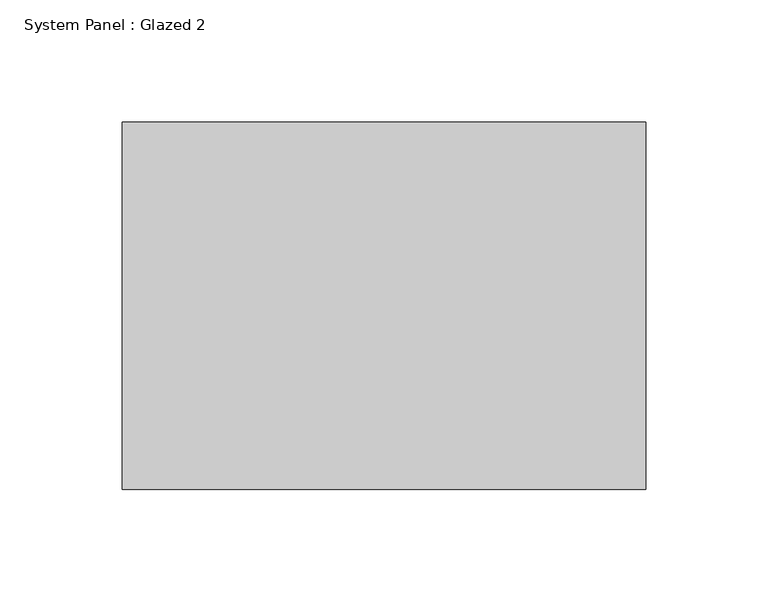
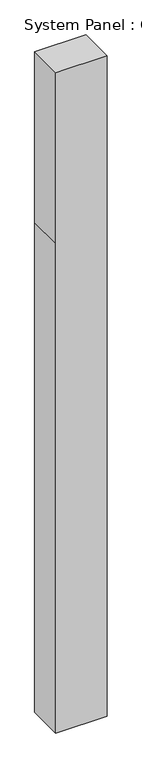
"""IFC4 building model written with IfcOpenShell, lengths in millimetres: plate geometry, System Panel : Glazed 2."""

import ifcopenshell
import ifcopenshell.guid

model = None  # the IFC model being written
_history = None  # IfcOwnerHistory: only IFC2X3 demands one
_inside = {}  # id of a spatial element -> (the spatial element, [elements in it])
_under = {}  # id of a project, library or spatial element -> (it, [spatial elements below it])
_declared = {}  # id of a project -> (the project, [libraries it declares])
_typed = {}  # id of a type object -> (the type object, [elements of that type])
_made_of = {}  # id of a material, layer set ... -> (it, [elements and type objects made of it])


def new_model(schema):
    """Start an empty IFC model of exactly this schema.

    Asked for "IFC4X3", IfcOpenShell would pick the latest addendum, in which some entities
    have other attributes; the version numbers below select the first issue.
    IFC2X3 requires an IfcOwnerHistory on every rooted entity: one is made here for all.
    """
    global model, _history
    if schema == "IFC4X3":
        model = ifcopenshell.file(schema_version=(4, 3, 0, 0))
    else:
        model = ifcopenshell.file(schema=schema)
    _inside.clear()
    _under.clear()
    _declared.clear()
    _typed.clear()
    _made_of.clear()
    _history = None
    if model.schema == "IFC2X3":
        org = make("IfcOrganization", Name="unknown")
        user = make(
            "IfcPersonAndOrganization",
            ThePerson=make("IfcPerson", FamilyName="unknown"),
            TheOrganization=org,
        )
        app = make(
            "IfcApplication",
            ApplicationDeveloper=org,
            Version="unknown",
            ApplicationFullName="unknown",
            ApplicationIdentifier="unknown",
        )
        _history = make(
            "IfcOwnerHistory",
            OwningUser=user,
            OwningApplication=app,
            ChangeAction="ADDED",
            CreationDate=0,
        )
    return model


def make(cls, **values):
    """One entity of the class cls with the attributes given. An attribute that is None is left unset."""
    return model.create_entity(
        cls, **{name: value for name, value in values.items() if value is not None}
    )


def rooted(cls, **values):
    """An entity with a GlobalId (a new one), such as an element, a storey or a relation."""
    return make(cls, GlobalId=ifcopenshell.guid.new(), OwnerHistory=_history, **values)


def si_unit(unit_type, name, prefix=None):
    """IfcSIUnit, for example si_unit("LENGTHUNIT", "METRE", prefix="MILLI")."""
    return make("IfcSIUnit", UnitType=unit_type, Prefix=prefix, Name=name)


def assignment(units):
    """IfcUnitAssignment: the units of a project."""
    return None if units is None else make("IfcUnitAssignment", Units=units)


def point(xyz):
    """IfcCartesianPoint."""
    return None if xyz is None else make("IfcCartesianPoint", Coordinates=xyz)


def direction(xyz):
    """IfcDirection."""
    return None if xyz is None else make("IfcDirection", DirectionRatios=xyz)


def frame(location, z_axis=None, x_axis=None):
    """IfcAxis2Placement3D, a coordinate frame: its origin and axes. An axis left out is left unset."""
    return make(
        "IfcAxis2Placement3D",
        Location=point(location),
        Axis=direction(z_axis),
        RefDirection=direction(x_axis),
    )


def origin():
    """The frame at (0, 0, 0) with its axes left unset."""
    return frame((0.0, 0.0, 0.0))


def place(relative_to, where):
    """IfcLocalPlacement: puts the frame where relative to a parent placement (None: the world)."""
    return make(
        "IfcLocalPlacement", PlacementRelTo=relative_to, RelativePlacement=where
    )


def context(
    kind, dimensions, precision=None, world=None, true_north=None, identifier=None
):
    """IfcGeometricRepresentationContext, for example the 3D "Model" context."""
    return make(
        "IfcGeometricRepresentationContext",
        ContextIdentifier=identifier,
        ContextType=kind,
        CoordinateSpaceDimension=dimensions,
        Precision=precision,
        WorldCoordinateSystem=world,
        TrueNorth=true_north,
    )


def project(units=None, contexts=None):
    """IfcProject with its units and contexts."""
    return rooted(
        "IfcProject",
        Name="project",
        RepresentationContexts=contexts,
        UnitsInContext=assignment(units),
    )


def spatial(cls, under=None, at=None, **own):
    """A site, building, storey or space (cls), placed at a placement, below another one or the project."""
    s = rooted(cls, ObjectPlacement=at, **own)
    if under is not None:
        _under.setdefault(under.id(), (under, []))[1].append(s)
    return s


def polyline(points):
    """IfcPolyline through the points."""
    return make("IfcPolyline", Points=[point(p) for p in points])


def outline(outer, holes=None, kind="AREA"):
    """IfcArbitraryClosedProfileDef: a profile drawn as a closed curve; with holes, ...WithVoids."""
    if holes is None:
        return make("IfcArbitraryClosedProfileDef", ProfileType=kind, OuterCurve=outer)
    return make(
        "IfcArbitraryProfileDefWithVoids",
        ProfileType=kind,
        OuterCurve=outer,
        InnerCurves=holes,
    )


def extrude(swept, where, along, depth):
    """IfcExtrudedAreaSolid: the profile swept, set in the frame where, extruded along a direction by depth."""
    return make(
        "IfcExtrudedAreaSolid",
        SweptArea=swept,
        Position=where,
        ExtrudedDirection=direction(along),
        Depth=depth,
    )


def shape(context_of_items, identifier, shape_type, items):
    """IfcShapeRepresentation: the items that make up one representation, for example the "Body"."""
    return make(
        "IfcShapeRepresentation",
        ContextOfItems=context_of_items,
        RepresentationIdentifier=identifier,
        RepresentationType=shape_type,
        Items=items,
    )


def source(mapping_origin, context_of_items, identifier, shape_type, items):
    """IfcRepresentationMap: a shape defined once, which mapped items show again and again."""
    return make(
        "IfcRepresentationMap",
        MappingOrigin=mapping_origin,
        MappedRepresentation=shape(context_of_items, identifier, shape_type, items),
    )


def transform(
    local_origin,
    x_axis=None,
    y_axis=None,
    z_axis=None,
    scale=None,
    scale2=None,
    scale3=None,
    uniform=True,
):
    """IfcCartesianTransformationOperator3D, or its non-uniform kind. x_axis, y_axis, z_axis: its Axis1, 2, 3."""
    if uniform:
        return make(
            "IfcCartesianTransformationOperator3D",
            Axis1=direction(x_axis),
            Axis2=direction(y_axis),
            LocalOrigin=point(local_origin),
            Scale=scale,
            Axis3=direction(z_axis),
        )
    return make(
        "IfcCartesianTransformationOperator3DnonUniform",
        Axis1=direction(x_axis),
        Axis2=direction(y_axis),
        LocalOrigin=point(local_origin),
        Scale=scale,
        Axis3=direction(z_axis),
        Scale2=scale2,
        Scale3=scale3,
    )


def mapped(mapping_source, mapping_target):
    """IfcMappedItem: shows the shape of a source again, moved by a transform."""
    return make(
        "IfcMappedItem", MappingSource=mapping_source, MappingTarget=mapping_target
    )


def made_of(thing, what):
    """Note that an element or type object is made of a material, layer set ...; save() writes the relation."""
    if what is not None:
        _made_of.setdefault(what.id(), (what, []))[1].append(thing)
    return thing


def element(
    cls,
    number,
    at=None,
    inside=None,
    cuts=None,
    type_object=None,
    material=None,
    context=None,
    identifier="Body",
    shape_type=None,
    held_by="IfcProductDefinitionShape",
    body=None,
    shapes=None,
    **own,
):
    """One element of the class cls, such as IfcWall. Its Tag is "e" and its number.

    at: its placement. inside: the storey or other place that contains it. cuts: it is an
    opening in that element (IfcRelVoidsElement). A single representation is given by context,
    identifier, shape_type and body (its items); several are given by shapes. held_by: the class
    of the entity that holds the representations. save() writes the other relations.
    """
    e = rooted(cls, Tag="e%d" % number, ObjectPlacement=at, **own)
    if body is not None:
        shapes = [shape(context, identifier, shape_type, body)]
    if shapes is not None:
        e.Representation = make(held_by, Representations=shapes)
    if inside is not None:
        _inside.setdefault(inside.id(), (inside, []))[1].append(e)
    if cuts is not None:
        rooted(
            "IfcRelVoidsElement", RelatingBuildingElement=cuts, RelatedOpeningElement=e
        )
    if type_object is not None:
        _typed.setdefault(type_object.id(), (type_object, []))[1].append(e)
    return made_of(e, material)


def aggregate(whole, parts):
    """IfcRelAggregates: a whole, such as a stair, and the parts it consists of."""
    return rooted("IfcRelAggregates", RelatingObject=whole, RelatedObjects=parts)


def save(model, path):
    """Write the relations noted so far, then the file.

    IfcRelAggregates (storeys below a building ...), IfcRelContainedInSpatialStructure (elements
    in a storey), IfcRelDefinesByType, IfcRelAssociatesMaterial and IfcRelDeclares: one each for
    every whole, place, type object, material and project.
    """
    for whole, parts in _under.values():
        aggregate(whole, parts)
    for where, things in _inside.values():
        rooted(
            "IfcRelContainedInSpatialStructure",
            RelatedElements=things,
            RelatingStructure=where,
        )
    for kind, things in _typed.values():
        rooted("IfcRelDefinesByType", RelatedObjects=things, RelatingType=kind)
    for what, things in _made_of.values():
        rooted("IfcRelAssociatesMaterial", RelatedObjects=things, RelatingMaterial=what)
    for by, libraries in _declared.values():
        rooted("IfcRelDeclares", RelatingContext=by, RelatedDefinitions=libraries)
    model.write(path)


def system_panel_glazed_2_22e75d95(model_context):
    return source(origin(), model_context, "Body", "SweptSolid", [
        extrude(outline(polyline([(0.0, -106.8917232), (0.0, 106.8917232), (2150.0, 106.8917232), (2900.0, 106.8917232), (2900.0, -106.8917232), (2150.0, -106.8917232), (0.0, -106.8917232)])), frame((0.0, -75.0, 0.0), z_axis=(0.0, 1.0, 0.0), x_axis=(0.0, 0.0, 1.0)), (0.0, 0.0, 1.0), 150.0),
    ])


if __name__ == "__main__":
    model = new_model("IFC4")
    model_context = context("Model", 3, world=origin())
    ifc_project = project(units=[si_unit("LENGTHUNIT", "METRE", prefix="MILLI")], contexts=[model_context])
    site = spatial("IfcSite", under=ifc_project)
    building = spatial("IfcBuilding", under=site)
    placement = place(None, origin())
    system_panel_glazed_2_shape = system_panel_glazed_2_22e75d95(model_context)
    element("IfcPlate", 1, ObjectType="System Panel : Glazed 2", at=placement, inside=building, context=model_context, shape_type="MappedRepresentation", body=[
        mapped(system_panel_glazed_2_shape, transform((0.0, 0.0, 0.0), x_axis=(1.0, 0.0, 0.0), y_axis=(0.0, 1.0, 0.0), z_axis=(0.0, 0.0, 1.0))),
    ])
    save(model, "model.ifc")

# Revit data of these elements
# Type "System Panel : Glazed 2"
#   COBie.Type = no
# Element 1 (IfcPlate, "System Panel : Glazed 2")
#   Materials on its faces: "Glass"
# Materials
#   "Glass": class "Glass", colour RGB 0 128 192, transparency 0.75, Description = "Soda Lime Glass", Cost = 0
